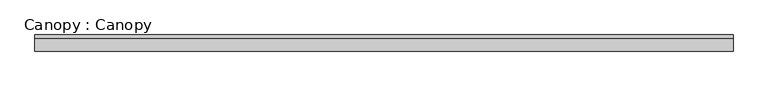
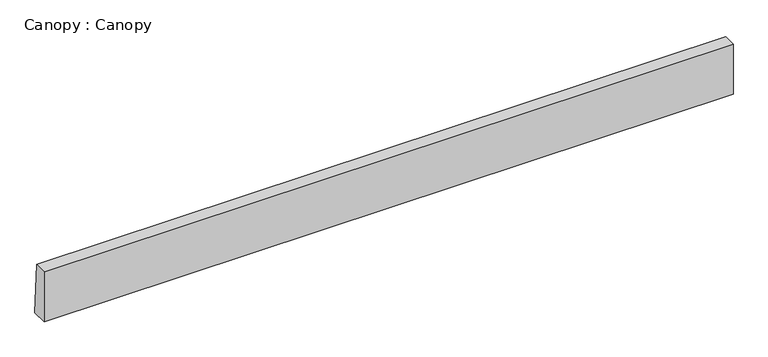
"""IFC4 building model written with IfcOpenShell, lengths in millimetres: proxy geometry, Canopy : Canopy."""

import ifcopenshell
import ifcopenshell.guid

model = None  # the IFC model being written
_history = None  # IfcOwnerHistory: only IFC2X3 demands one
_inside = {}  # id of a spatial element -> (the spatial element, [elements in it])
_under = {}  # id of a project, library or spatial element -> (it, [spatial elements below it])
_declared = {}  # id of a project -> (the project, [libraries it declares])
_typed = {}  # id of a type object -> (the type object, [elements of that type])
_made_of = {}  # id of a material, layer set ... -> (it, [elements and type objects made of it])


def new_model(schema):
    """Start an empty IFC model of exactly this schema.

    Asked for "IFC4X3", IfcOpenShell would pick the latest addendum, in which some entities
    have other attributes; the version numbers below select the first issue.
    IFC2X3 requires an IfcOwnerHistory on every rooted entity: one is made here for all.
    """
    global model, _history
    if schema == "IFC4X3":
        model = ifcopenshell.file(schema_version=(4, 3, 0, 0))
    else:
        model = ifcopenshell.file(schema=schema)
    _inside.clear()
    _under.clear()
    _declared.clear()
    _typed.clear()
    _made_of.clear()
    _history = None
    if model.schema == "IFC2X3":
        org = make("IfcOrganization", Name="unknown")
        user = make(
            "IfcPersonAndOrganization",
            ThePerson=make("IfcPerson", FamilyName="unknown"),
            TheOrganization=org,
        )
        app = make(
            "IfcApplication",
            ApplicationDeveloper=org,
            Version="unknown",
            ApplicationFullName="unknown",
            ApplicationIdentifier="unknown",
        )
        _history = make(
            "IfcOwnerHistory",
            OwningUser=user,
            OwningApplication=app,
            ChangeAction="ADDED",
            CreationDate=0,
        )
    return model


def make(cls, **values):
    """One entity of the class cls with the attributes given. An attribute that is None is left unset."""
    return model.create_entity(
        cls, **{name: value for name, value in values.items() if value is not None}
    )


def rooted(cls, **values):
    """An entity with a GlobalId (a new one), such as an element, a storey or a relation."""
    return make(cls, GlobalId=ifcopenshell.guid.new(), OwnerHistory=_history, **values)


def si_unit(unit_type, name, prefix=None):
    """IfcSIUnit, for example si_unit("LENGTHUNIT", "METRE", prefix="MILLI")."""
    return make("IfcSIUnit", UnitType=unit_type, Prefix=prefix, Name=name)


def assignment(units):
    """IfcUnitAssignment: the units of a project."""
    return None if units is None else make("IfcUnitAssignment", Units=units)


def point(xyz):
    """IfcCartesianPoint."""
    return None if xyz is None else make("IfcCartesianPoint", Coordinates=xyz)


def direction(xyz):
    """IfcDirection."""
    return None if xyz is None else make("IfcDirection", DirectionRatios=xyz)


def frame(location, z_axis=None, x_axis=None):
    """IfcAxis2Placement3D, a coordinate frame: its origin and axes. An axis left out is left unset."""
    return make(
        "IfcAxis2Placement3D",
        Location=point(location),
        Axis=direction(z_axis),
        RefDirection=direction(x_axis),
    )


def origin():
    """The frame at (0, 0, 0) with its axes left unset."""
    return frame((0.0, 0.0, 0.0))


def place(relative_to, where):
    """IfcLocalPlacement: puts the frame where relative to a parent placement (None: the world)."""
    return make(
        "IfcLocalPlacement", PlacementRelTo=relative_to, RelativePlacement=where
    )


def context(
    kind, dimensions, precision=None, world=None, true_north=None, identifier=None
):
    """IfcGeometricRepresentationContext, for example the 3D "Model" context."""
    return make(
        "IfcGeometricRepresentationContext",
        ContextIdentifier=identifier,
        ContextType=kind,
        CoordinateSpaceDimension=dimensions,
        Precision=precision,
        WorldCoordinateSystem=world,
        TrueNorth=true_north,
    )


def project(units=None, contexts=None):
    """IfcProject with its units and contexts."""
    return rooted(
        "IfcProject",
        Name="project",
        RepresentationContexts=contexts,
        UnitsInContext=assignment(units),
    )


def spatial(cls, under=None, at=None, **own):
    """A site, building, storey or space (cls), placed at a placement, below another one or the project."""
    s = rooted(cls, ObjectPlacement=at, **own)
    if under is not None:
        _under.setdefault(under.id(), (under, []))[1].append(s)
    return s


def polyline(points):
    """IfcPolyline through the points."""
    return make("IfcPolyline", Points=[point(p) for p in points])


def outline(outer, holes=None, kind="AREA"):
    """IfcArbitraryClosedProfileDef: a profile drawn as a closed curve; with holes, ...WithVoids."""
    if holes is None:
        return make("IfcArbitraryClosedProfileDef", ProfileType=kind, OuterCurve=outer)
    return make(
        "IfcArbitraryProfileDefWithVoids",
        ProfileType=kind,
        OuterCurve=outer,
        InnerCurves=holes,
    )


def extrude(swept, where, along, depth):
    """IfcExtrudedAreaSolid: the profile swept, set in the frame where, extruded along a direction by depth."""
    return make(
        "IfcExtrudedAreaSolid",
        SweptArea=swept,
        Position=where,
        ExtrudedDirection=direction(along),
        Depth=depth,
    )


def shape(context_of_items, identifier, shape_type, items):
    """IfcShapeRepresentation: the items that make up one representation, for example the "Body"."""
    return make(
        "IfcShapeRepresentation",
        ContextOfItems=context_of_items,
        RepresentationIdentifier=identifier,
        RepresentationType=shape_type,
        Items=items,
    )


def source(mapping_origin, context_of_items, identifier, shape_type, items):
    """IfcRepresentationMap: a shape defined once, which mapped items show again and again."""
    return make(
        "IfcRepresentationMap",
        MappingOrigin=mapping_origin,
        MappedRepresentation=shape(context_of_items, identifier, shape_type, items),
    )


def transform(
    local_origin,
    x_axis=None,
    y_axis=None,
    z_axis=None,
    scale=None,
    scale2=None,
    scale3=None,
    uniform=True,
):
    """IfcCartesianTransformationOperator3D, or its non-uniform kind. x_axis, y_axis, z_axis: its Axis1, 2, 3."""
    if uniform:
        return make(
            "IfcCartesianTransformationOperator3D",
            Axis1=direction(x_axis),
            Axis2=direction(y_axis),
            LocalOrigin=point(local_origin),
            Scale=scale,
            Axis3=direction(z_axis),
        )
    return make(
        "IfcCartesianTransformationOperator3DnonUniform",
        Axis1=direction(x_axis),
        Axis2=direction(y_axis),
        LocalOrigin=point(local_origin),
        Scale=scale,
        Axis3=direction(z_axis),
        Scale2=scale2,
        Scale3=scale3,
    )


def mapped(mapping_source, mapping_target):
    """IfcMappedItem: shows the shape of a source again, moved by a transform."""
    return make(
        "IfcMappedItem", MappingSource=mapping_source, MappingTarget=mapping_target
    )


def made_of(thing, what):
    """Note that an element or type object is made of a material, layer set ...; save() writes the relation."""
    if what is not None:
        _made_of.setdefault(what.id(), (what, []))[1].append(thing)
    return thing


def element(
    cls,
    number,
    at=None,
    inside=None,
    cuts=None,
    type_object=None,
    material=None,
    context=None,
    identifier="Body",
    shape_type=None,
    held_by="IfcProductDefinitionShape",
    body=None,
    shapes=None,
    **own,
):
    """One element of the class cls, such as IfcWall. Its Tag is "e" and its number.

    at: its placement. inside: the storey or other place that contains it. cuts: it is an
    opening in that element (IfcRelVoidsElement). A single representation is given by context,
    identifier, shape_type and body (its items); several are given by shapes. held_by: the class
    of the entity that holds the representations. save() writes the other relations.
    """
    e = rooted(cls, Tag="e%d" % number, ObjectPlacement=at, **own)
    if body is not None:
        shapes = [shape(context, identifier, shape_type, body)]
    if shapes is not None:
        e.Representation = make(held_by, Representations=shapes)
    if inside is not None:
        _inside.setdefault(inside.id(), (inside, []))[1].append(e)
    if cuts is not None:
        rooted(
            "IfcRelVoidsElement", RelatingBuildingElement=cuts, RelatedOpeningElement=e
        )
    if type_object is not None:
        _typed.setdefault(type_object.id(), (type_object, []))[1].append(e)
    return made_of(e, material)


def aggregate(whole, parts):
    """IfcRelAggregates: a whole, such as a stair, and the parts it consists of."""
    return rooted("IfcRelAggregates", RelatingObject=whole, RelatedObjects=parts)


def save(model, path):
    """Write the relations noted so far, then the file.

    IfcRelAggregates (storeys below a building ...), IfcRelContainedInSpatialStructure (elements
    in a storey), IfcRelDefinesByType, IfcRelAssociatesMaterial and IfcRelDeclares: one each for
    every whole, place, type object, material and project.
    """
    for whole, parts in _under.values():
        aggregate(whole, parts)
    for where, things in _inside.values():
        rooted(
            "IfcRelContainedInSpatialStructure",
            RelatedElements=things,
            RelatingStructure=where,
        )
    for kind, things in _typed.values():
        rooted("IfcRelDefinesByType", RelatedObjects=things, RelatingType=kind)
    for what, things in _made_of.values():
        rooted("IfcRelAssociatesMaterial", RelatedObjects=things, RelatingMaterial=what)
    for by, libraries in _declared.values():
        rooted("IfcRelDeclares", RelatingContext=by, RelatedDefinitions=libraries)
    model.write(path)


def canopy_canopy_d66d4a18(model_context):
    return source(origin(), model_context, "Body", "SweptSolid", [
        extrude(outline(polyline([(150.0, 0.0), (0.0, 0.0), (0.0, 500.0), (120.0, 500.0), (150.0, 0.0)])), frame((-3250.0, 0.0, 0.0), z_axis=(1.0, 0.0, 0.0), x_axis=(0.0, 1.0, 0.0)), (0.0, 0.0, 1.0), 6500.0),
    ])


if __name__ == "__main__":
    model = new_model("IFC4")
    model_context = context("Model", 3, world=origin())
    ifc_project = project(units=[si_unit("LENGTHUNIT", "METRE", prefix="MILLI")], contexts=[model_context])
    site = spatial("IfcSite", under=ifc_project)
    building = spatial("IfcBuilding", under=site)
    placement = place(None, origin())
    canopy_canopy_shape = canopy_canopy_d66d4a18(model_context)
    element("IfcBuildingElementProxy", 1, Name="Canopy : Canopy", ObjectType="Canopy : Canopy", at=placement, inside=building, context=model_context, shape_type="MappedRepresentation", body=[
        mapped(canopy_canopy_shape, transform((0.0, 0.0, 0.0), x_axis=(1.0, 0.0, 0.0), y_axis=(0.0, 1.0, 0.0), z_axis=(0.0, 0.0, 1.0))),
    ])
    save(model, "model.ifc")

# Revit data of these elements
# Type "Canopy : Canopy"
#   Type Comments = "CV-AG"
#   H_Rebar Ratio = 0.1
#   Canopy Width [instance default] = 1700 mm
#   Canopy Length [instance default] = 1000 mm
#   Canopy L.P = 120 mm
#   Canopy H.P = 150 mm
#   구조재료 = Concrete_f'c=28MPa(Cylender)
#   Default Elevation = 0
# Element 1 (IfcBuildingElementProxy, "Canopy : Canopy")
#   Canopy Width = 6500 mm
#   Canopy Length = 500 mm
#   Materials on its faces: "Concrete_f'c=28MPa(Cylender)"
# Materials
#   "Concrete_f'c=28MPa(Cylender)": class "Concrete", colour RGB 176 176 176, transparency 0, Description = "Reinf. Conc.", Cost = 0, Image = Concrete.Cast-In-Place.Flat.Polished.Grey.jpg
